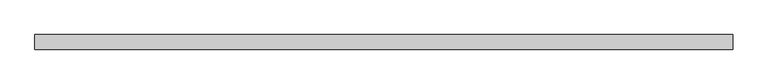
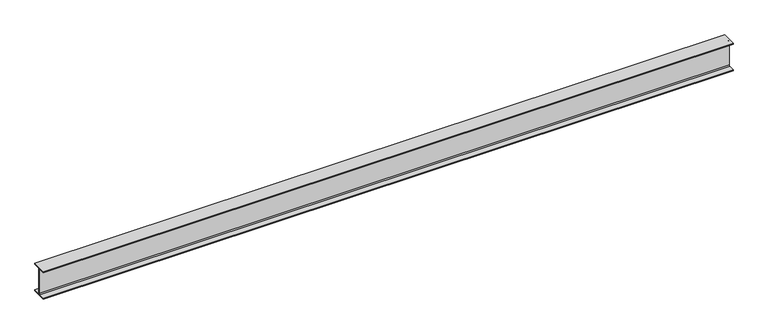
"""IFC4 building model written with IfcOpenShell, lengths in millimetres: beam geometry, 0912_Steel Framing_H-KSD3502 : H_SB_ASB_H-400x200x8x13."""

from ifc_helpers import new_model, si_unit, point, frame, frame_2d, origin, place, context, project, spatial, polyline, circle_curve, trimmed, segment, composite_curve, outline, extrude, source, transform, mapped, element, save


def beam_2daac4a0(model_context):
    return source(origin(), model_context, "Body", "SweptSolid", [
        extrude(outline(composite_curve([segment(polyline([(100.0, -187.0), (100.0, -200.0), (-100.0, -200.0), (-100.0, -187.0), (-20.0, -187.0)]), True, "CONTINUOUS"), segment(trimmed(circle_curve(frame_2d((-20.0, -171.0)), 16.0), [point((-20.0, -187.0))], [point((-4.0, -171.0))], True, "CARTESIAN"), True, "CONTINUOUS"), segment(polyline([(-4.0, -171.0), (-4.0, 171.0)]), True, "CONTINUOUS"), segment(trimmed(circle_curve(frame_2d((-20.0, 171.0)), 16.0), [point((-4.0, 171.0))], [point((-20.0, 187.0))], True, "CARTESIAN"), True, "CONTINUOUS"), segment(polyline([(-20.0, 187.0), (-100.0, 187.0), (-100.0, 200.0), (100.0, 200.0), (100.0, 187.0), (20.0, 187.0)]), True, "CONTINUOUS"), segment(trimmed(circle_curve(frame_2d((20.0, 171.0)), 16.0), [point((20.0, 187.0))], [point((4.0, 171.0))], True, "CARTESIAN"), True, "CONTINUOUS"), segment(polyline([(4.0, 171.0), (4.0, -171.0)]), True, "CONTINUOUS"), segment(trimmed(circle_curve(frame_2d((20.0, -171.0)), 16.0), [point((4.0, -171.0))], [point((20.0, -187.0))], True, "CARTESIAN"), True, "CONTINUOUS"), segment(polyline([(20.0, -187.0), (100.0, -187.0)]), True, "CONTINUOUS")], self_intersect=False)), frame((-4664.4729123, 0.0, 0.0), z_axis=(1.0, 0.0, 0.0), x_axis=(0.0, 1.0, 0.0)), (0.0, 0.0, 1.0), 9526.7729123),
    ])


if __name__ == "__main__":
    model = new_model("IFC4")
    model_context = context("Model", 3, world=origin())
    ifc_project = project(units=[si_unit("LENGTHUNIT", "METRE", prefix="MILLI")], contexts=[model_context])
    site = spatial("IfcSite", under=ifc_project)
    building = spatial("IfcBuilding", under=site)
    placement = place(None, origin())
    beam_shape = beam_2daac4a0(model_context)
    element("IfcBeam", 1, ObjectType="0912_Steel Framing_H-KSD3502 : H_SB_ASB_H-400x200x8x13", at=placement, inside=building, context=model_context, shape_type="MappedRepresentation", body=[
        mapped(beam_shape, transform((0.0, 0.0, 0.0), x_axis=(1.0, 0.0, 0.0), y_axis=(0.0, 1.0, 0.0), z_axis=(0.0, 0.0, 1.0))),
    ])
    save(model, "model.ifc")

# Revit data of these elements
# Type "0912_Steel Framing_H-KSD3502 : H_SB_ASB_H-400x200x8x13"
#   H_WM Code_1 = "S01AA002-00001 | Main Steel Structure Fabrication Work | Shelter/Building | Medium Steel - Standard (90KG/M>Weight≥30KG/M) | Material: (   )"
#   H_WM Code_2 = "S03AA028-00001 | Main Steel Structure Erection Work | Shelter/Building | Medium Steel (90KG/M>Weight≥30KG/M) | Material: (   )"
#   H_WM Code_3 = "S01AA010-00001 | Main Steel Structure Fabrication Work | Shelter/Building | Steel Painting/Coating | for Non-Fireproofed Steel Surface, Surface Preparation, Primer, Second & Final Coat | Material: (   )"
#   H_Q'ty Cal Type Tag = "SB-Q2"
#   Width = 20.0 cm
#   Web Thickness = 0.8 cm
#   Web Fillet = 1.6 cm
#   Warping Constant = 649000.0 cm⁶
#   W = 0
#   Torsional Moment of Inertia = 35.8981 cm⁴
#   Section Area = 84.12 cm²
#   Plastic Modulus weak axis = 268.0 cm³
#   Plastic Modulus strong axis = 1330.0 cm³
#   Perimeter = 1.56 m²/m
#   Nominal Weight = 66.00 kgf/m
#   Moment of Inertia weak axis = 1740.00 cm⁴
#   Moment of Inertia strong axis = 23700.00 cm⁴
#   Height = 40.0 cm
#   Flange Thickness = 1.3 cm
#   Elastic Modulus weak axis = 174.0 cm³
#   Elastic Modulus strong axis = 1190.0 cm³
#   Centroid Vertical = 20.0 cm
#   Centroid Horizontal = 10.0 cm
#   Ix = 237000000
#   Length [instance default] = 1.5240 m
#   Zx = 1330000
#   b = 0.2000 m
#   h = 0.4000 m
#   r = 0.0160 m
#   s = 0.0080 m
#   t = 0.0130 m
#   A = 0.008412 m²
#   Structural Material [instance default] = Steel, 45-345
#   Assembly Code = ""
# Element 1 (IfcBeam, "0912_Steel Framing_H-KSD3502 : H_SB_ASB_H-400x200x8x13")
#   Structural Material = none
# Materials
#   "Steel, 45-345": class "Metal", colour RGB 189 187 185, transparency 0, Description = "Steel 345 MPa", Cost = 0
